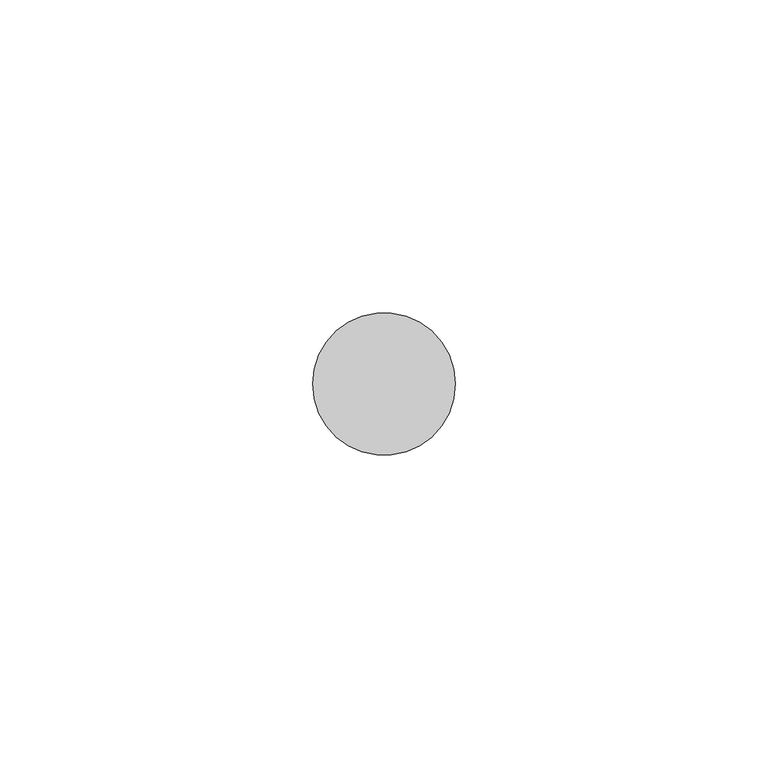
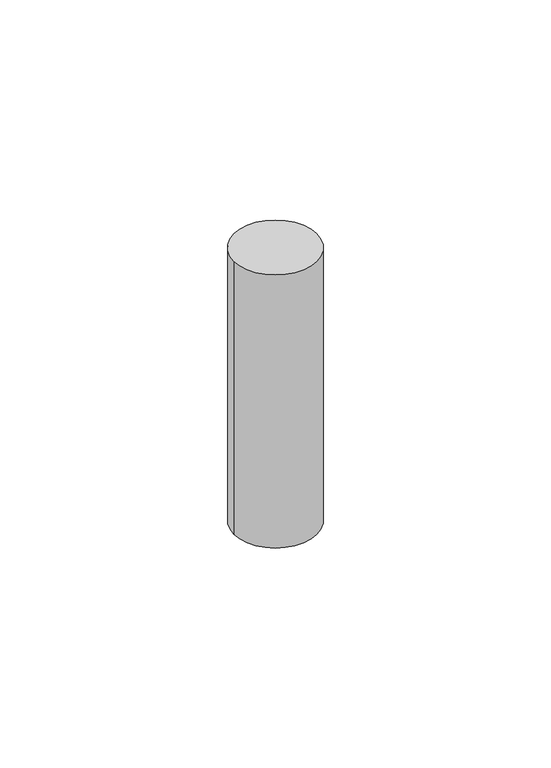
"""IFC4 building model written with IfcOpenShell, lengths in millimetres: proxy geometry, Bolt18:Bolt003:304655 : Bolt18:Bolt003:304655."""

from ifc_helpers import new_model, si_unit, point, frame, frame_2d, origin, place, context, project, spatial, circle_curve, trimmed, segment, composite_curve, outline, extrude, source, transform, mapped, element, save


def generic_models_0087d09a(model_context):
    return source(origin(), model_context, "Body", "SweptSolid", [
        extrude(outline(composite_curve([segment(trimmed(circle_curve(frame_2d((9839.3437094, 2276.5207483)), 11.4045168), [point((9850.7482262, 2276.5207483))], [point((9827.9391926, 2276.5207483))], False, "CARTESIAN"), True, "CONTINUOUS"), segment(trimmed(circle_curve(frame_2d((9839.3437094, 2276.5207483)), 11.4045168), [point((9827.9391926, 2276.5207483))], [point((9850.7482262, 2276.5207483))], False, "CARTESIAN"), True, "CONTINUOUS")], self_intersect=False)), frame((0.0, 0.0, 36645.5959962), z_axis=(0.0, 0.0, 1.0), x_axis=(1.0, 0.0, 0.0)), (0.0, 0.0, 1.0), 79.375),
    ])


if __name__ == "__main__":
    model = new_model("IFC4")
    model_context = context("Model", 3, world=origin())
    ifc_project = project(units=[si_unit("LENGTHUNIT", "METRE", prefix="MILLI")], contexts=[model_context])
    site = spatial("IfcSite", under=ifc_project)
    building = spatial("IfcBuilding", under=site)
    placement = place(None, origin())
    generic_models_shape = generic_models_0087d09a(model_context)
    element("IfcBuildingElementProxy", 1, Name="Bolt18:Bolt003:304655 : Bolt18:Bolt003:304655", ObjectType="Bolt18:Bolt003:304655 : Bolt18:Bolt003:304655", at=placement, inside=building, context=model_context, shape_type="MappedRepresentation", body=[
        mapped(generic_models_shape, transform((0.0, 0.0, 0.0), x_axis=(1.0, 0.0, 0.0), y_axis=(0.0, 1.0, 0.0), z_axis=(0.0, 0.0, 1.0))),
    ])
    save(model, "model.ifc")

# Revit data of these elements
# Type "Bolt18:Bolt003:304655 : Bolt18:Bolt003:304655"
#   NameOverride = "Bolt18:Bolt003:304655"
#   ObjectTypeOverride = "Bolt18:Bolt003"
#   Reference = "Bolt003"
#   Category = "Generic Models"
#   Tag = "304655"
# Element 1 (IfcBuildingElementProxy, "Bolt18:Bolt003:304655 : Bolt18:Bolt003:304655")
#   Materials on its faces: "TUBE STEEL STRINGER WELDED TO ANCHORED STEEL PLATE - SEE STRUCT DWGS"
# Materials
#   "TUBE STEEL STRINGER WELDED TO ANCHORED STEEL PLATE - SEE STRUCT DWGS": class "Unassigned", colour RGB 128 128 128, transparency 0, Cost = 0
